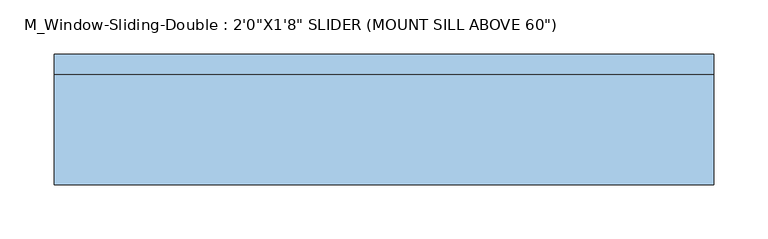
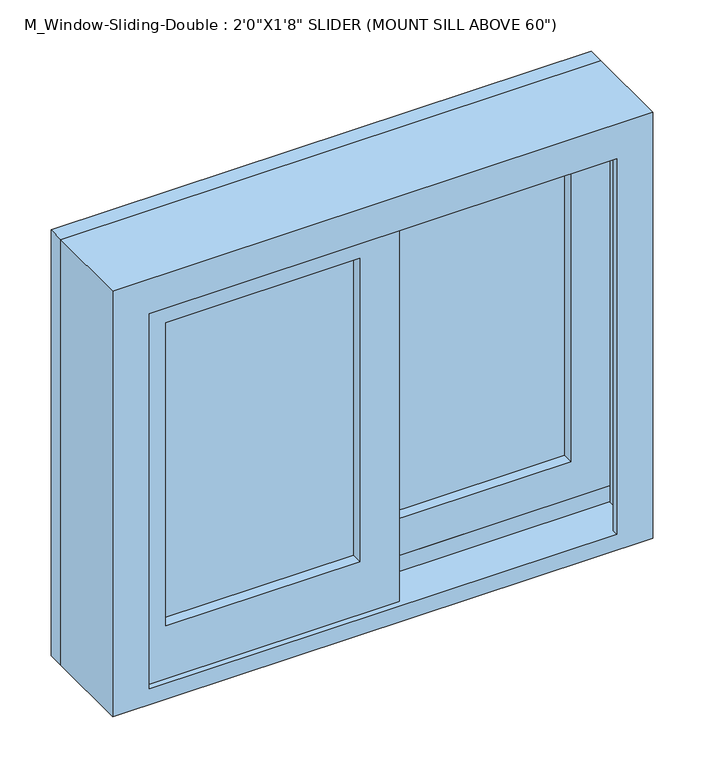
"""IFC4 building model written with IfcOpenShell, lengths in millimetres: window geometry."""

from ifc_helpers import new_model, si_unit, frame, origin, place, context, project, spatial, polyline, outline, extrude, faceted_brep, source, transform, mapped, element, save


def window_704dc0b4(model_context):
    return source(origin(), model_context, "Body", "SolidModel", [
        faceted_brep([(-304.8, 35.56, 900.0), (304.8, 35.56, 900.0), (304.8, -66.04, 900.0), (-304.8, -66.04, 900.0), (-263.8778905, -66.04, 1367.0778905), (-263.8778905, -66.04, 919.05), (-263.8778905, -59.69, 919.05), (-263.8778905, -59.69, 1367.0778905), (-285.75, -59.69, 919.05), (-285.75, -59.69, 1388.95), (285.75, -59.69, 1388.95), (285.75, -59.69, 919.05), (263.8778905, -59.69, 919.05), (263.8778905, -59.69, 1367.0778905), (-285.75, -15.24, 919.05), (-285.75, -15.24, 938.1), (-285.75, 29.21, 938.1), (-285.75, 29.21, 919.05), (-285.75, 35.56, 919.05), (-285.75, 35.56, 1388.95), (-304.8, 35.56, 1408.0), (304.8, 35.56, 1408.0), (285.75, 35.56, 1388.95), (285.75, 35.56, 919.05), (-304.8, -66.04, 1408.0), (304.8, -66.04, 1408.0), (263.8778905, -66.04, 1367.0778905), (263.8778905, -66.04, 919.05), (285.75, 29.21, 919.05), (285.75, 29.21, 938.1), (285.75, -15.24, 938.1), (285.75, -15.24, 919.05)], [[[0, 1, 2, 3]], [[4, 5, 6, 7]], [[7, 6, 8, 9, 10, 11, 12, 13]], [[9, 8, 14, 15, 16, 17, 18, 19]], [[0, 20, 21, 1], [22, 19, 18, 23]], [[24, 20, 0, 3]], [[2, 25, 24, 3], [4, 26, 27, 5]], [[7, 13, 26, 4]], [[9, 19, 22, 10]], [[20, 24, 25, 21]], [[13, 12, 27, 26]], [[22, 23, 28, 29, 30, 31, 11, 10]], [[21, 25, 2, 1]], [[27, 12, 11, 31, 14, 8, 6, 5]], [[31, 30, 15, 14]], [[30, 29, 16, 15]], [[29, 28, 17, 16]], [[18, 17, 28, 23]]]),
        extrude(outline(polyline([(1408.0, 304.8), (1408.0, -304.8), (900.0, -304.8), (900.0, 304.8), (1408.0, 304.8)]), holes=[polyline([(1388.95, -285.75), (1388.95, 285.75), (919.05, 285.75), (919.05, -285.75), (1388.95, -285.75)])]), frame((0.0, 35.56, 0.0), z_axis=(0.0, 1.0, 0.0), x_axis=(0.0, 0.0, 1.0)), (0.0, 0.0, 1.0), 19.05),
        extrude(outline(polyline([(241.3, -2.54), (22.225, -2.54), (22.225, 3.81), (241.3, 3.81), (241.3, -2.54)])), frame((0.0, 0.0, 982.55), z_axis=(0.0, 0.0, 1.0), x_axis=(1.0, 0.0, 0.0)), (0.0, 0.0, 1.0), 361.95),
        extrude(outline(polyline([(241.3, 10.16), (22.225, 10.16), (22.225, 16.51), (241.3, 16.51), (241.3, 10.16)])), frame((0.0, 0.0, 982.55), z_axis=(0.0, 0.0, 1.0), x_axis=(1.0, 0.0, 0.0)), (0.0, 0.0, 1.0), 361.95),
        extrude(outline(polyline([(-22.225, -46.99), (-241.3, -46.99), (-241.3, -40.64), (-22.225, -40.64), (-22.225, -46.99)])), frame((0.0, 0.0, 982.55), z_axis=(0.0, 0.0, 1.0), x_axis=(1.0, 0.0, 0.0)), (0.0, 0.0, 1.0), 361.95),
        extrude(outline(polyline([(-22.225, -34.29), (-241.3, -34.29), (-241.3, -27.94), (-22.225, -27.94), (-22.225, -34.29)])), frame((0.0, 0.0, 982.55), z_axis=(0.0, 0.0, 1.0), x_axis=(1.0, 0.0, 0.0)), (0.0, 0.0, 1.0), 361.95),
        extrude(outline(polyline([(919.05, 22.225), (1388.95, 22.225), (1388.95, -285.75), (919.05, -285.75), (919.05, 22.225)]), holes=[polyline([(1344.5, -241.3), (1344.5, -22.225), (982.55, -22.225), (982.55, -241.3), (1344.5, -241.3)])]), frame((0.0, -59.69, 0.0), z_axis=(0.0, 1.0, 0.0), x_axis=(0.0, 0.0, 1.0)), (0.0, 0.0, 1.0), 44.45),
        extrude(outline(polyline([(938.1, -22.225), (938.1, 285.75), (1388.95, 285.75), (1388.95, -22.225), (938.1, -22.225)]), holes=[polyline([(982.55, 241.3), (982.55, 22.225), (1344.5, 22.225), (1344.5, 241.3), (982.55, 241.3)])]), frame((0.0, -15.24, 0.0), z_axis=(0.0, 1.0, 0.0), x_axis=(0.0, 0.0, 1.0)), (0.0, 0.0, 1.0), 44.45),
    ])


if __name__ == "__main__":
    model = new_model("IFC4")
    model_context = context("Model", 3, world=origin())
    ifc_project = project(units=[si_unit("LENGTHUNIT", "METRE", prefix="MILLI")], contexts=[model_context])
    site = spatial("IfcSite", under=ifc_project)
    building = spatial("IfcBuilding", under=site)
    placement = place(None, origin())
    window_shape = window_704dc0b4(model_context)
    element("IfcWindow", 1, ObjectType="M_Window-Sliding-Double : 2'0\"X1'8\" SLIDER (MOUNT SILL ABOVE 60\")", at=placement, inside=building, context=model_context, shape_type="MappedRepresentation", body=[
        mapped(window_shape, transform((0.0, 0.0, 0.0), x_axis=(1.0, 0.0, 0.0), y_axis=(0.0, 1.0, 0.0), z_axis=(0.0, 0.0, 1.0))),
    ])
    save(model, "model.ifc")

# Revit data of these elements
# Type "M_Window-Sliding-Double : 2'0\"X1'8\" SLIDER (MOUNT SILL ABOVE 60\")"
#   Type Mark = "1"
#   Fire Rating = "0.5h"
#   Assembly Code = "B2020100"
#   Analytic Construction = "Double glazing - domestic"
#   Window Inset [instance default] = 0' - 0"
#   Wall Thickness [instance default] = 0' - 5.90551"
#   Visual Light Transmittance = 0.81
#   Thermal Resistance (R) = 1.8146 (h·ft²·°F)/BTU
#   Solar Heat Gain Coefficient = 0.76
#   Muntin Width = 0' - 8 5/8"
#   Muntin Height = 1' - 2 1/4"
#   Interior Wall Closure [instance default] = 0' - 2.65551"
#   Heat Transfer Coefficient (U) = 0.5511 BTU/(h·ft²·°F)
#   Frame Extension [instance default] = 0' - 0 1/4"
#   Exterior Wall Closure [instance default] = 0' - 1 1/4"
#   Rough Width = 2' - 0.59055"
#   Rough Height = 1' - 8.59055"
#   Height = 1' - 8"
#   Extension Jamb [instance default] = 0' - 2.65551"
#   Default Sill Height = 2' - 11.43307"
#   Width = 2' - 0"
#   Interior Trim Visibility [instance default] = yes
#   Indicator Visibility [instance default] = yes
#   Exterior Trim Visibility [instance default] = yes
#   Muntin Visibility = yes
#   Extension Jamb Visibility [instance default] = yes
#   Muntin Pattern = M_Muntin Pattern_2x2 : M_Muntin Pattern_2x2
#   Interior Trim Material = Wood - Stained
#   Interior Trim = M_Trim-Window-Interior-Flat : Picture Frame
#   Interior Frame Material = Wood - Stained
#   Glass Panel Material = Glass
#   Exterior Trim Material = Clad - White
#   Exterior Trim = M_Trim-Window-Exterior-Flat : with Sill
#   Exterior Frame Material = Clad - White
#   Wall Closure = (empty or 0)
# Element 1 (IfcWindow, "M_Window-Sliding-Double : 2'0\"X1'8\" SLIDER (MOUNT SILL ABOVE 60\")")
#   Wall Thickness = 0' - 4"
#   Extension Jamb = 0' - 0 3/4"
#   Materials on its faces: "Wood - Stained", "Glass", "Clad - White"
# Materials
#   "Wood - Stained": class "Wood", colour RGB 224 178 126, transparency 0, Cost = 0
#   "Glass": class "Glass", colour RGB 0 128 192, transparency 0.75, Description = "Soda Lime Glass", Cost = 0
#   "Clad - White": class "Wood", colour RGB 242 242 238, transparency 0, Cost = 0
